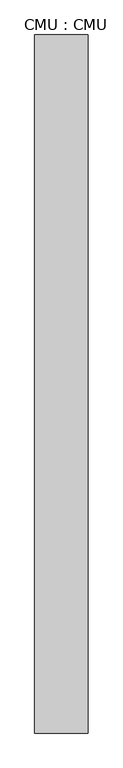
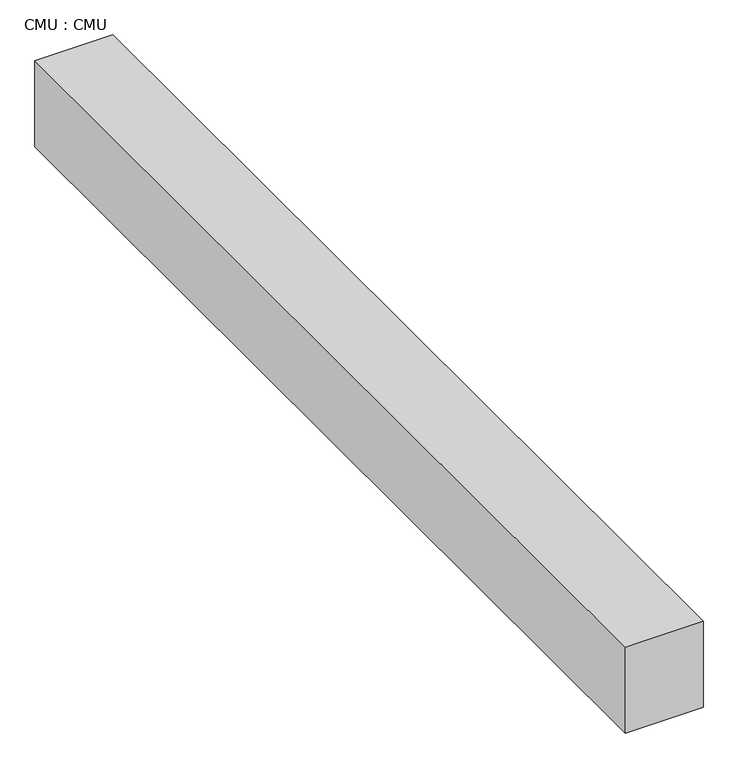
"""IFC4 building model written with IfcOpenShell, lengths in millimetres: proxy geometry, CMU : CMU."""

from ifc_helpers import new_model, si_unit, frame, origin, place, context, project, spatial, polyline, outline, extrude, source, transform, mapped, element, save


def cmu_cmu_2291ce66(model_context):
    return source(origin(), model_context, "Body", "SweptSolid", [
        extrude(outline(polyline([(-10098.4737014, 7982.1531721), (-10250.8737014, 7982.1531721), (-10250.8737014, 9982.1531721), (-10098.4737014, 9982.1531721), (-10098.4737014, 7982.1531721)])), frame((0.0, 0.0, 33196.2086935), z_axis=(0.0, 0.0, 1.0), x_axis=(1.0, 0.0, 0.0)), (0.0, 0.0, 1.0), 177.8),
    ])


if __name__ == "__main__":
    model = new_model("IFC4")
    model_context = context("Model", 3, world=origin())
    ifc_project = project(units=[si_unit("LENGTHUNIT", "METRE", prefix="MILLI")], contexts=[model_context])
    site = spatial("IfcSite", under=ifc_project)
    building = spatial("IfcBuilding", under=site)
    placement = place(None, origin())
    cmu_cmu_shape = cmu_cmu_2291ce66(model_context)
    element("IfcBuildingElementProxy", 1, Name="CMU : CMU", ObjectType="CMU : CMU", at=placement, inside=building, context=model_context, shape_type="MappedRepresentation", body=[
        mapped(cmu_cmu_shape, transform((0.0, 0.0, 0.0), x_axis=(1.0, 0.0, 0.0), y_axis=(0.0, 1.0, 0.0), z_axis=(0.0, 0.0, 1.0))),
    ])
    save(model, "model.ifc")

# Revit data of these elements
# Type "CMU : CMU"
#   NameOverride = "CMU"
# Element 1 (IfcBuildingElementProxy, "CMU : CMU")
#   Materials on its faces: "4\" CMU WALL"
# Materials
#   "4\" CMU WALL": class "Unassigned", colour RGB 128 128 128, transparency 0, Cost = 0
